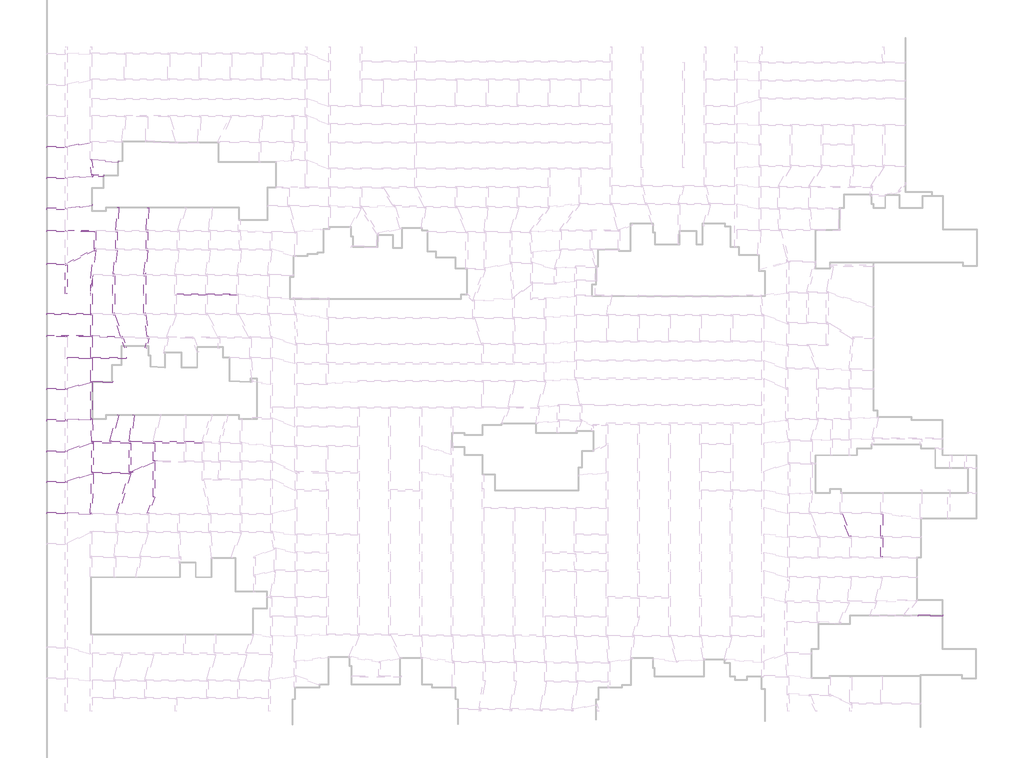
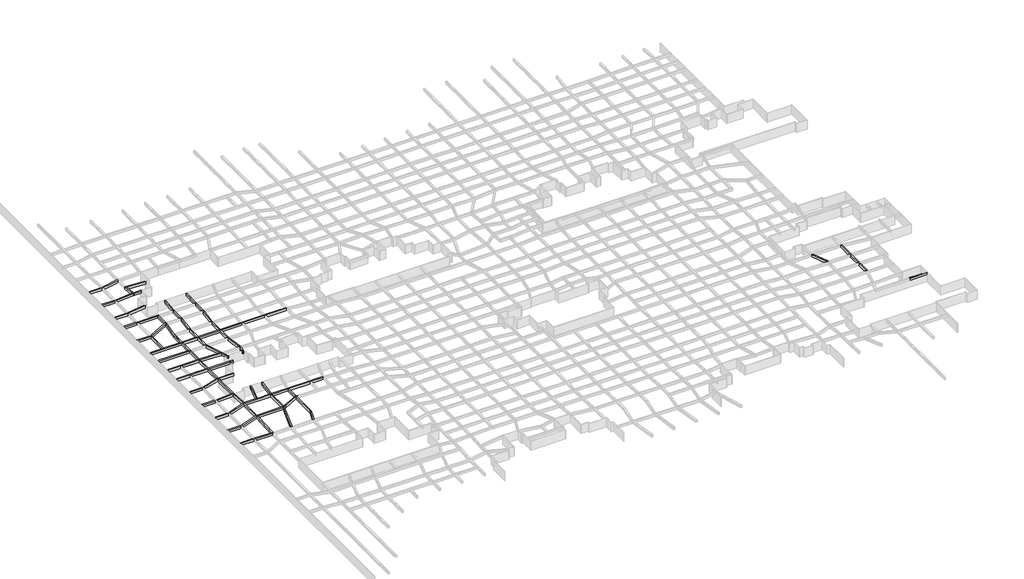
# One storey, part 25 of 45: 64 beams.
"""IFC4 building model written with IfcOpenShell, lengths in millimetres."""

from ifc_helpers import new_model, si_unit, frame, origin, place, context, project, spatial, polyline, outline, extrude, faceted_brep, element, save

model = new_model("IFC4")

# Units and contexts
model_context = context("Model", 3, world=origin())
ifc_project = project(units=[si_unit("LENGTHUNIT", "METRE", prefix="MILLI")], contexts=[model_context])

# Site, building, storey
site = spatial("IfcSite", under=ifc_project)
building = spatial("IfcBuilding", under=site)
storey = spatial("IfcBuildingStorey", under=building, Name="户型图", Elevation=0.0)

# Beams
placement = place(None, origin())
element("IfcBeam", 1, ObjectType="混凝土 - 矩形梁 : KL_beam", at=placement, inside=storey, context=model_context, shape_type="SweptSolid", body=[
    extrude(outline(polyline([(-155040.1872489, 93329.932653), (-155040.1872489, 93729.932653), (-150359.8528414, 93729.932653), (-150359.8528414, 93329.932653), (-155040.1872489, 93329.932653)])), frame((0.0, 0.0, 2500.0), z_axis=(0.0, 0.0, 1.0), x_axis=(1.0, 0.0, 0.0)), (0.0, 0.0, 1.0), 800.0),
])
element("IfcBeam", 2, ObjectType="混凝土 - 矩形梁 : KL_beam", at=placement, inside=storey, context=model_context, shape_type="SweptSolid", body=[
    extrude(outline(polyline([(-155040.1872489, 85529.932653), (-155040.1872489, 85929.932653), (-150359.8528414, 85929.932653), (-150359.8528414, 85529.932653), (-155040.1872489, 85529.932653)])), frame((0.0, 0.0, 2500.0), z_axis=(0.0, 0.0, 1.0), x_axis=(1.0, 0.0, 0.0)), (0.0, 0.0, 1.0), 800.0),
])
element("IfcBeam", 3, ObjectType="混凝土 - 矩形梁 : KL_beam", at=placement, inside=storey, context=model_context, shape_type="SweptSolid", body=[
    extrude(outline(polyline([(-155040.1872489, 77829.932653), (-155040.1872489, 78229.932653), (-150359.8528414, 78229.932653), (-150359.8528414, 77829.932653), (-155040.1872489, 77829.932653)])), frame((0.0, 0.0, 2500.0), z_axis=(0.0, 0.0, 1.0), x_axis=(1.0, 0.0, 0.0)), (0.0, 0.0, 1.0), 800.0),
])
element("IfcBeam", 4, ObjectType="混凝土 - 矩形梁 : KL_beam", at=placement, inside=storey, context=model_context, shape_type="SweptSolid", body=[
    extrude(outline(polyline([(-155040.1872489, 72229.932653), (-155040.1872489, 72629.932653), (-150359.8528414, 72629.932653), (-150359.8528414, 72229.932653), (-155040.1872489, 72229.932653)])), frame((0.0, 0.0, 2500.0), z_axis=(0.0, 0.0, 1.0), x_axis=(1.0, 0.0, 0.0)), (0.0, 0.0, 1.0), 800.0),
])
element("IfcBeam", 5, ObjectType="混凝土 - 矩形梁 : KL_beam", at=placement, inside=storey, context=model_context, shape_type="SweptSolid", body=[
    extrude(outline(polyline([(-155040.1872489, 63929.9626201), (-155040.1872489, 64329.9626201), (-150359.8528414, 64329.9626201), (-150359.8528414, 63929.9626201), (-155040.1872489, 63929.9626201)])), frame((0.0, 0.0, 2500.0), z_axis=(0.0, 0.0, 1.0), x_axis=(1.0, 0.0, 0.0)), (0.0, 0.0, 1.0), 800.0),
])
element("IfcBeam", 6, ObjectType="混凝土 - 矩形梁 : KL_beam", at=placement, inside=storey, context=model_context, shape_type="Brep", body=[
    faceted_brep([(-149959.8528414, 64456.5033467, 3300.0), (-149959.8528414, 64007.5728516, 3300.0), (-143187.4265839, 67458.2963847, 3300.0), (-142895.0186512, 67607.285668, 3300.0), (-142743.034403, 67684.7255104, 3300.0), (-142743.034403, 68007.285668, 3300.0), (-142743.034403, 68133.6560054, 3300.0), (-143143.034403, 67929.8458256, 3300.0), (-149959.8528414, 64007.5728516, 2500.0), (-143187.4265839, 67458.2963847, 2500.0), (-142895.0186512, 67607.285668, 2500.0), (-142743.034403, 67684.7255104, 2500.0), (-149959.8528414, 64456.5033467, 2500.0), (-143143.034403, 67929.8458256, 2500.0), (-142743.034403, 68133.6560054, 2500.0), (-142743.034403, 68007.285668, 2500.0)], [[[0, 1, 2, 3, 4, 5, 6, 7]], [[1, 8, 9, 10, 11, 4, 3, 2]], [[8, 12, 13, 14, 15, 11, 10, 9]], [[6, 14, 13, 12, 0, 7]], [[0, 12, 8, 1]], [[6, 5, 4, 11, 15, 14]]]),
    faceted_brep([(-150359.8528414, 63929.9626201, 3300.0), (-150112.1714971, 63929.9626201, 3300.0), (-150112.1714971, 63929.9626201, 2500.0), (-150359.8528414, 63929.9626201, 2500.0), (-150359.8528414, 63803.7626718, 2500.0), (-150359.8528414, 63803.7626718, 3300.0)], [[[0, 1, 2, 3]], [[4, 5, 0, 3]], [[1, 0, 5]], [[2, 1, 5, 4]], [[3, 2, 4]]]),
])
element("IfcBeam", 7, ObjectType="混凝土 - 矩形梁 : KL_beam", at=placement, inside=storey, context=model_context, shape_type="Brep", body=[
    faceted_brep([(-142743.034403, 72229.932653, 3300.0), (-142743.034403, 72629.6091605, 3300.0), (-142743.034403, 72629.932653, 3300.0), (-149959.8528414, 72629.932653, 3300.0), (-149959.8528414, 72229.932653, 3300.0), (-143143.034403, 72229.932653, 3300.0), (-142743.034403, 72229.932653, 2500.0), (-149959.8528414, 72229.932653, 2500.0), (-143143.034403, 72229.932653, 2500.0), (-142743.034403, 72629.932653, 2500.0), (-142743.034403, 72629.6091605, 2500.0), (-149959.8528414, 72629.932653, 2500.0)], [[[0, 1, 2, 3, 4, 5]], [[6, 0, 5, 4, 7, 8]], [[9, 10, 6, 8, 7, 11]], [[2, 9, 11, 3]], [[4, 3, 11, 7]], [[2, 1, 0, 6, 10, 9]]]),
])
element("IfcBeam", 8, ObjectType="混凝土 - 矩形梁 : KL_beam", at=placement, inside=storey, context=model_context, shape_type="Brep", body=[
    faceted_brep([(-143143.034403, 67929.8458256, 3300.0), (-142743.034403, 68133.6560054, 3300.0), (-142743.034403, 72229.6091605, 3300.0), (-142743.034403, 72229.932653, 3300.0), (-143143.034403, 72229.932653, 3300.0), (-142743.034403, 68133.6560054, 2500.0), (-142743.034403, 72229.6091605, 2500.0), (-142743.034403, 72229.932653, 2500.0), (-143143.034403, 67929.8458256, 2500.0), (-143143.034403, 72229.932653, 2500.0)], [[[0, 1, 2, 3, 4]], [[1, 5, 6, 7, 3, 2]], [[5, 8, 9, 7, 6]], [[8, 0, 4, 9]], [[1, 0, 8, 5]], [[4, 3, 7, 9]]]),
])
element("IfcBeam", 9, ObjectType="混凝土 - 矩形梁 : KL_beam", at=placement, inside=storey, context=model_context, shape_type="SweptSolid", body=[
    extrude(outline(polyline([(-137343.034403, 68007.285668), (-137743.034403, 68007.285668), (-137743.034403, 72229.6091605), (-137343.034403, 72229.6091605), (-137343.034403, 68007.285668)])), frame((0.0, 0.0, 2500.0), z_axis=(0.0, 0.0, 1.0), x_axis=(1.0, 0.0, 0.0)), (0.0, 0.0, 1.0), 800.0),
])
element("IfcBeam", 10, ObjectType="混凝土 - 矩形梁 : KL_beam", at=placement, inside=storey, context=model_context, shape_type="SweptSolid", body=[
    extrude(outline(polyline([(-129643.034403, 68007.285668), (-130043.034403, 68007.285668), (-130043.034403, 72229.6091605), (-129643.034403, 72229.6091605), (-129643.034403, 68007.285668)])), frame((0.0, 0.0, 2500.0), z_axis=(0.0, 0.0, 1.0), x_axis=(1.0, 0.0, 0.0)), (0.0, 0.0, 1.0), 800.0),
])
element("IfcBeam", 11, ObjectType="混凝土 - 矩形梁 : KL_beam", at=placement, inside=storey, context=model_context, shape_type="SweptSolid", body=[
    extrude(outline(polyline([(-129837.0055379, 78332.9949392), (-129437.249207, 78319.0351406), (-129635.9283402, 72629.6091605), (-130036.172158, 72629.6091605), (-129837.0055379, 78332.9949392)])), frame((0.0, 0.0, 2500.0), z_axis=(0.0, 0.0, 1.0), x_axis=(1.0, 0.0, 0.0)), (0.0, 0.0, 1.0), 800.0),
])
element("IfcBeam", 12, ObjectType="混凝土 - 矩形梁 : KL_beam", at=placement, inside=storey, context=model_context, shape_type="SweptSolid", body=[
    extrude(outline(polyline([(-137324.0083706, 78428.9447568), (-136924.9827505, 78401.0421673), (-137328.560661, 72629.6091605), (-137729.5374202, 72629.6091605), (-137324.0083706, 78428.9447568)])), frame((0.0, 0.0, 2500.0), z_axis=(0.0, 0.0, 1.0), x_axis=(1.0, 0.0, 0.0)), (0.0, 0.0, 1.0), 800.0),
])
element("IfcBeam", 13, ObjectType="混凝土 - 矩形梁 : KL_beam", at=placement, inside=storey, context=model_context, shape_type="SweptSolid", body=[
    extrude(outline(polyline([(-143652.5805457, 79146.4826455), (-143596.9113053, 78750.375418), (-149959.8528414, 77856.1223033), (-149959.8528414, 78260.0533323), (-143652.5805457, 79146.4826455)])), frame((0.0, 0.0, 2500.0), z_axis=(0.0, 0.0, 1.0), x_axis=(1.0, 0.0, 0.0)), (0.0, 0.0, 1.0), 800.0),
])
element("IfcBeam", 14, ObjectType="混凝土 - 矩形梁 : KL_beam", at=placement, inside=storey, context=model_context, shape_type="Brep", body=[
    faceted_brep([(-143368.2977458, 86123.352764, 3300.0), (-143401.7015992, 86505.1605551, 3300.0), (-143403.1600429, 86521.8306433, 3300.0), (-143801.6379222, 86486.9683462, 3300.0), (-149959.8528414, 85948.1943532, 3300.0), (-149959.8528414, 85546.6664182, 3300.0), (-143576.2356454, 86105.1605551, 3300.0), (-143368.2977458, 86123.352764, 2500.0), (-149959.8528414, 85546.6664182, 2500.0), (-143576.2356454, 86105.1605551, 2500.0), (-143403.1600429, 86521.8306433, 2500.0), (-143401.7015992, 86505.1605551, 2500.0), (-149959.8528414, 85948.1943532, 2500.0), (-143801.6379222, 86486.9683462, 2500.0)], [[[0, 1, 2, 3, 4, 5, 6]], [[7, 0, 6, 5, 8, 9]], [[10, 11, 7, 9, 8, 12, 13]], [[2, 10, 13, 12, 4, 3]], [[5, 4, 12, 8]], [[2, 1, 0, 7, 11, 10]]]),
])
element("IfcBeam", 15, ObjectType="混凝土 - 矩形梁 : KL_beam", at=placement, inside=storey, context=model_context, shape_type="Brep", body=[
    faceted_brep([(-143749.2394727, 90477.5366261, 3300.0), (-144133.590805, 90443.9102418, 3300.0), (-144147.7173519, 90442.674329, 3300.0), (-143801.6379222, 86486.9683462, 3300.0), (-143403.1600429, 86521.8306433, 3300.0), (-143713.9426126, 90074.09167, 3300.0), (-143749.2394727, 90477.5366261, 2500.0), (-143403.1600429, 86521.8306433, 2500.0), (-143713.9426126, 90074.09167, 2500.0), (-144147.7173519, 90442.674329, 2500.0), (-144133.590805, 90443.9102418, 2500.0), (-143801.6379222, 86486.9683462, 2500.0)], [[[0, 1, 2, 3, 4, 5]], [[6, 0, 5, 4, 7, 8]], [[9, 10, 6, 8, 7, 11]], [[2, 9, 11, 3]], [[4, 3, 11, 7]], [[2, 1, 0, 6, 10, 9]]]),
])
element("IfcBeam", 16, ObjectType="混凝土 - 矩形梁 : KL_beam", at=placement, inside=storey, context=model_context, shape_type="Brep", body=[
    faceted_brep([(-137036.4475634, 90008.1324887, 3300.0), (-137064.3501529, 89609.1068686, 3300.0), (-137064.3501529, 89609.1068686, 2500.0), (-137036.4475634, 90008.1324887, 2500.0), (-143733.590805, 90476.4423647, 3300.0), (-143749.2394727, 90477.5366261, 3300.0), (-143713.9426126, 90074.09167, 3300.0), (-143713.9426126, 90074.09167, 2500.0), (-143749.2394727, 90477.5366261, 2500.0), (-143733.590805, 90476.4423647, 2500.0)], [[[0, 1, 2, 3]], [[1, 0, 4, 5, 6]], [[2, 1, 6, 7]], [[3, 2, 7, 8, 9]], [[0, 3, 9, 8, 5, 4]], [[6, 5, 8, 7]]]),
])
element("IfcBeam", 17, ObjectType="混凝土 - 矩形梁 : KL_beam", at=placement, inside=storey, context=model_context, shape_type="SweptSolid", body=[
    extrude(outline(polyline([(-149959.8528414, 93365.130378), (-149959.8528414, 93772.617056), (-144133.590805, 94905.1276718), (-144133.590805, 94497.6409938), (-149959.8528414, 93365.130378)])), frame((0.0, 0.0, 2500.0), z_axis=(0.0, 0.0, 1.0), x_axis=(1.0, 0.0, 0.0)), (0.0, 0.0, 1.0), 800.0),
])
element("IfcBeam", 18, ObjectType="混凝土 - 矩形梁 : KL_beam", at=placement, inside=storey, context=model_context, shape_type="SweptSolid", body=[
    extrude(outline(polyline([(-140684.967834, 86505.1605551), (-140684.967834, 86105.1605551), (-143576.2356454, 86105.1605551), (-143368.2977458, 86123.352764), (-143401.7015992, 86505.1605551), (-140684.967834, 86505.1605551)])), frame((0.0, 0.0, 2500.0), z_axis=(0.0, 0.0, 1.0), x_axis=(1.0, 0.0, 0.0)), (0.0, 0.0, 1.0), 800.0),
])
element("IfcBeam", 19, ObjectType="混凝土 - 矩形梁 : KL_beam", at=placement, inside=storey, context=model_context, shape_type="SweptSolid", body=[
    extrude(outline(polyline([(-137765.00064, 67607.285668), (-137362.8299892, 67607.285668), (-137992.6084803, 61570.3096597), (-138394.779131, 61570.3096597), (-137765.00064, 67607.285668)])), frame((0.0, 0.0, 2500.0), z_axis=(0.0, 0.0, 1.0), x_axis=(1.0, 0.0, 0.0)), (0.0, 0.0, 1.0), 800.0),
])
element("IfcBeam", 20, ObjectType="混凝土 - 矩形梁 : KL_beam", at=placement, inside=storey, context=model_context, shape_type="Brep", body=[
    faceted_brep([(-129662.8131158, 67607.285668, 3300.0), (-130064.9837666, 67607.285668, 3300.0), (-130694.7622577, 61570.3096597, 3300.0), (-130292.5916069, 61570.3096597, 3300.0), (-130266.1701137, 61823.5827117, 3300.0), (-130064.9837666, 67607.285668, 2500.0), (-130694.7622577, 61570.3096597, 2500.0), (-129662.8131158, 67607.285668, 2500.0), (-130266.1701137, 61823.5827117, 2500.0), (-130292.5916069, 61570.3096597, 2500.0)], [[[0, 1, 2, 3, 4]], [[1, 5, 6, 2]], [[5, 7, 8, 9, 6]], [[7, 0, 4, 3, 9, 8]], [[1, 0, 7, 5]], [[3, 2, 6, 9]]]),
])
element("IfcBeam", 21, ObjectType="混凝土 - 矩形梁 : KL_beam", at=placement, inside=storey, context=model_context, shape_type="Brep", body=[
    faceted_brep([(-130292.5916069, 61570.3096597, 3300.0), (-130266.1701137, 61570.3096597, 3300.0), (-130266.1701137, 61823.5827117, 3300.0), (-130266.1701137, 61570.3096597, 2500.0), (-130266.1701137, 61823.5827117, 2500.0), (-130292.5916069, 61570.3096597, 2500.0)], [[[0, 1, 2]], [[1, 3, 4, 2]], [[3, 5, 4]], [[3, 1, 0, 5]], [[0, 2, 4, 5]]]),
    faceted_brep([(-130266.1701137, 61170.3096597, 3300.0), (-130266.1701137, 61170.3096597, 2500.0), (-130334.3196833, 61170.3096597, 2500.0), (-130666.1701137, 61170.3096597, 2500.0), (-130666.1701137, 61170.3096597, 3300.0), (-130334.3196833, 61170.3096597, 3300.0), (-130666.1701137, 56692.8612022, 3300.0), (-130666.1701137, 56292.8612022, 3300.0), (-130666.1701137, 51854.9299556, 3300.0), (-130266.1701137, 51854.9299556, 3300.0), (-130266.1701137, 56292.8612022, 3300.0), (-130266.1701137, 56692.8612022, 3300.0), (-130266.1701137, 51854.9299556, 2500.0), (-130266.1701137, 56292.8612022, 2500.0), (-130266.1701137, 56692.8612022, 2500.0), (-130666.1701137, 51854.9299556, 2500.0), (-130666.1701137, 56292.8612022, 2500.0), (-130666.1701137, 56692.8612022, 2500.0)], [[[0, 1, 2, 3, 4, 5]], [[5, 4, 6, 7, 8, 9, 10, 11, 0]], [[1, 0, 11, 10, 9, 12, 13, 14]], [[2, 1, 14, 13, 12, 15, 16, 17, 3]], [[4, 3, 17, 16, 15, 8, 7, 6]], [[9, 8, 15, 12]]]),
])
element("IfcBeam", 22, ObjectType="混凝土 - 矩形梁 : KL_beam", at=placement, inside=storey, context=model_context, shape_type="Brep", body=[
    faceted_brep([(-138030.1531976, 61170.3096597, 3300.0), (-138430.1531976, 61170.3096597, 3300.0), (-138430.1531976, 56692.8612022, 3300.0), (-138430.1531976, 56292.8612022, 3300.0), (-138430.1531976, 51854.9299556, 3300.0), (-138030.1531976, 51854.9299556, 3300.0), (-138030.1531976, 56292.8612022, 3300.0), (-138030.1531976, 56692.8612022, 3300.0), (-138030.1531976, 61170.3096597, 2500.0), (-138030.1531976, 51854.9299556, 2500.0), (-138030.1531976, 56292.8612022, 2500.0), (-138030.1531976, 56692.8612022, 2500.0), (-138430.1531976, 61170.3096597, 2500.0), (-138430.1531976, 51854.9299556, 2500.0), (-138430.1531976, 56292.8612022, 2500.0), (-138430.1531976, 56692.8612022, 2500.0)], [[[0, 1, 2, 3, 4, 5, 6, 7]], [[8, 0, 7, 6, 5, 9, 10, 11]], [[12, 8, 11, 10, 9, 13, 14, 15]], [[1, 12, 15, 14, 13, 4, 3, 2]], [[1, 0, 8, 12]], [[5, 4, 13, 9]]]),
])
element("IfcBeam", 23, ObjectType="混凝土 - 矩形梁 : KL_beam", at=placement, inside=storey, context=model_context, shape_type="Brep", body=[
    faceted_brep([(-144029.1794601, 51454.5502515, 2500.0), (-144029.1794601, 51454.5502515, 3300.0), (-144029.1794601, 51854.5502515, 3300.0), (-144029.1794601, 56292.8612022, 3300.0), (-144029.1794601, 56692.8612022, 3300.0), (-144029.1794601, 57320.5657345, 3300.0), (-144029.1794601, 57320.5657345, 2500.0), (-144029.1794601, 56692.8612022, 2500.0), (-144029.1794601, 56292.8612022, 2500.0), (-144029.1794601, 51854.5502515, 2500.0), (-143629.1794601, 51454.5502515, 3300.0), (-143629.1794601, 51454.5502515, 2500.0), (-143629.1794601, 51454.9299556, 3300.0), (-143629.1794601, 51854.9299556, 3300.0), (-143629.1794601, 56292.8612022, 3300.0), (-143629.1794601, 56692.8612022, 3300.0), (-143629.1794601, 60578.3043057, 3300.0), (-143629.1794601, 51454.9299556, 2500.0), (-143629.1794601, 51854.9299556, 2500.0), (-143629.1794601, 56292.8612022, 2500.0), (-143629.1794601, 56692.8612022, 2500.0), (-143629.1794601, 60578.3043057, 2500.0)], [[[0, 1, 2, 3, 4, 5, 6, 7, 8, 9]], [[10, 1, 0, 11]], [[1, 10, 12, 13, 14, 15, 16, 5, 4, 3, 2]], [[10, 11, 17, 18, 19, 20, 21, 16, 15, 14, 13, 12]], [[11, 0, 9, 8, 7, 6, 21, 20, 19, 18, 17]], [[6, 5, 16, 21]]]),
])
element("IfcBeam", 24, ObjectType="混凝土 - 矩形梁 : KL_beam", at=placement, inside=storey, context=model_context, shape_type="Brep", body=[
    faceted_brep([(-155040.3480617, 56292.8612022, 3300.0), (-155040.3480617, 56692.8612022, 3300.0), (-155040.3480617, 56692.8612022, 2500.0), (-155040.3480617, 56292.8612022, 2500.0), (-144029.1794601, 56292.8612022, 3300.0), (-144029.1794601, 56692.8612022, 3300.0), (-149959.8528414, 56692.8612022, 3300.0), (-150359.8528414, 56692.8612022, 3300.0), (-144029.1794601, 56692.8612022, 2500.0), (-149959.8528414, 56692.8612022, 2500.0), (-150359.8528414, 56692.8612022, 2500.0), (-144029.1794601, 56292.8612022, 2500.0)], [[[0, 1, 2, 3]], [[1, 0, 4, 5, 6, 7]], [[2, 1, 7, 6, 5, 8, 9, 10]], [[3, 2, 10, 9, 8, 11]], [[0, 3, 11, 4]], [[5, 4, 11, 8]]]),
    faceted_brep([(-107154.3480617, 56292.8612022, 3300.0), (-107154.3480617, 56292.8612022, 2500.0), (-107154.3480617, 56670.8773262, 2500.0), (-107154.3480617, 56692.8612022, 2500.0), (-107154.3480617, 56692.8612022, 3300.0), (-107154.3480617, 56670.8773262, 3300.0), (-122502.1870297, 56292.8612022, 3300.0), (-122502.1870297, 56692.8612022, 3300.0), (-122502.1870297, 56692.8612022, 2500.0), (-122502.1870297, 56292.8612022, 2500.0), (-114728.2029549, 56692.8612022, 3300.0), (-115128.2029549, 56692.8612022, 3300.0), (-115128.2029549, 56292.8612022, 3300.0), (-114728.2029549, 56292.8612022, 3300.0), (-107385.8902631, 56292.8612022, 3300.0), (-114728.2029549, 56692.8612022, 2500.0), (-115128.2029549, 56692.8612022, 2500.0), (-107385.8902631, 56292.8612022, 2500.0), (-114728.2029549, 56292.8612022, 2500.0), (-115128.2029549, 56292.8612022, 2500.0)], [[[0, 1, 2, 3, 4, 5]], [[6, 7, 8, 9]], [[0, 5, 4, 10, 11, 7, 6, 12, 13, 14]], [[4, 3, 15, 16, 8, 7, 11, 10]], [[3, 2, 1, 17, 18, 19, 9, 8, 16, 15]], [[1, 0, 14, 13, 12, 6, 9, 19, 18, 17]]]),
    faceted_brep([(-122902.1870297, 56692.8612022, 3300.0), (-122902.1870297, 56292.8612022, 3300.0), (-122902.1870297, 56292.8612022, 2500.0), (-122902.1870297, 56692.8612022, 2500.0), (-130266.1701137, 56292.8612022, 3300.0), (-130266.1701137, 56692.8612022, 3300.0), (-130266.1701137, 56692.8612022, 2500.0), (-130266.1701137, 56292.8612022, 2500.0)], [[[0, 1, 2, 3]], [[4, 5, 6, 7]], [[1, 0, 5, 4]], [[0, 3, 6, 5]], [[3, 2, 7, 6]], [[2, 1, 4, 7]]]),
    faceted_brep([(-130666.1701137, 56692.8612022, 3300.0), (-130666.1701137, 56292.8612022, 3300.0), (-130666.1701137, 56292.8612022, 2500.0), (-130666.1701137, 56692.8612022, 2500.0), (-138030.1531976, 56292.8612022, 3300.0), (-138030.1531976, 56692.8612022, 3300.0), (-138030.1531976, 56692.8612022, 2500.0), (-138030.1531976, 56292.8612022, 2500.0)], [[[0, 1, 2, 3]], [[4, 5, 6, 7]], [[1, 0, 5, 4]], [[0, 3, 6, 5]], [[3, 2, 7, 6]], [[2, 1, 4, 7]]]),
    faceted_brep([(-138430.1531976, 56692.8612022, 3300.0), (-138430.1531976, 56292.8612022, 3300.0), (-138430.1531976, 56292.8612022, 2500.0), (-138430.1531976, 56692.8612022, 2500.0), (-143629.1794601, 56292.8612022, 3300.0), (-143629.1794601, 56692.8612022, 3300.0), (-143629.1794601, 56692.8612022, 2500.0), (-143629.1794601, 56292.8612022, 2500.0)], [[[0, 1, 2, 3]], [[4, 5, 6, 7]], [[1, 0, 5, 4]], [[0, 3, 6, 5]], [[3, 2, 7, 6]], [[2, 1, 4, 7]]]),
])
element("IfcBeam", 25, ObjectType="混凝土 - 矩形梁 : KL_beam", at=placement, inside=storey, context=model_context, shape_type="SweptSolid", body=[
    extrude(outline(polyline([(-149959.8528414, 63929.9626201), (-149959.8528414, 56692.8612022), (-150359.8528414, 56692.8612022), (-150359.8528414, 63803.7626718), (-150112.1714971, 63929.9626201), (-149959.8528414, 63929.9626201)])), frame((0.0, 0.0, 2500.0), z_axis=(0.0, 0.0, 1.0), x_axis=(1.0, 0.0, 0.0)), (0.0, 0.0, 1.0), 800.0),
])
element("IfcBeam", 26, ObjectType="混凝土 - 矩形梁 : KL_beam", at=placement, inside=storey, context=model_context, shape_type="SweptSolid", body=[
    extrude(outline(polyline([(-155040.3505583, 51454.5502515), (-155040.3505583, 51854.5502515), (-144029.1794601, 51854.5502515), (-144029.1794601, 51454.5502515), (-155040.3505583, 51454.5502515)])), frame((0.0, 0.0, 2500.0), z_axis=(0.0, 0.0, 1.0), x_axis=(1.0, 0.0, 0.0)), (0.0, 0.0, 1.0), 800.0),
])
element("IfcBeam", 27, ObjectType="混凝土 - 矩形梁 : KL_beam", at=placement, inside=storey, context=model_context, shape_type="SweptSolid", body=[
    extrude(outline(polyline([(-130640.0234877, 51454.9299556), (-130236.0924587, 51454.9299556), (-129458.8661012, 45924.6770642), (-129862.7971302, 45924.6770642), (-130640.0234877, 51454.9299556)])), frame((0.0, 0.0, 2500.0), z_axis=(0.0, 0.0, 1.0), x_axis=(1.0, 0.0, 0.0)), (0.0, 0.0, 1.0), 800.0),
])
element("IfcBeam", 28, ObjectType="混凝土 - 矩形梁 : KL_beam", at=placement, inside=storey, context=model_context, shape_type="SweptSolid", body=[
    extrude(outline(polyline([(-135993.089329, 45924.6770642), (-136417.3284341, 45924.6770642), (-138371.532439, 51454.9299556), (-137947.2933339, 51454.9299556), (-135993.089329, 45924.6770642)])), frame((0.0, 0.0, 2500.0), z_axis=(0.0, 0.0, 1.0), x_axis=(1.0, 0.0, 0.0)), (0.0, 0.0, 1.0), 800.0),
])
element("IfcBeam", 29, ObjectType="混凝土 - 矩形梁 : KL_beam", at=placement, inside=storey, context=model_context, shape_type="Brep", body=[
    faceted_brep([(-144029.1794601, 25141.8814872, 3300.0), (-144018.8658517, 25142.5337653, 3300.0), (-143629.1794601, 25167.1792512, 3300.0), (-143629.1794601, 25366.7986539, 3300.0), (-143629.1794601, 34369.9375221, 3300.0), (-143629.1794601, 34769.9375221, 3300.0), (-143629.1794601, 40354.5502515, 3300.0), (-143629.1794601, 40754.5502515, 3300.0), (-143629.1794601, 45845.780438, 3300.0), (-143629.1794601, 46246.148229, 3300.0), (-143629.1794601, 51454.5502515, 3300.0), (-144029.1794601, 51454.5502515, 3300.0), (-144029.1794601, 46254.5502515, 3300.0), (-144029.1794601, 45854.5502515, 3300.0), (-144029.1794601, 40754.5502515, 3300.0), (-144029.1794601, 40354.5502515, 3300.0), (-144029.1794601, 34720.6483321, 3300.0), (-144029.1794601, 34304.5285578, 3300.0), (-144029.1794601, 25542.6806599, 3300.0), (-144029.1794601, 25141.8814872, 2500.0), (-144029.1794601, 51454.5502515, 2500.0), (-144029.1794601, 46254.5502515, 2500.0), (-144029.1794601, 45854.5502515, 2500.0), (-144029.1794601, 40754.5502515, 2500.0), (-144029.1794601, 40354.5502515, 2500.0), (-144029.1794601, 34720.6483321, 2500.0), (-144029.1794601, 34304.5285578, 2500.0), (-144029.1794601, 25542.6806599, 2500.0), (-143629.1794601, 25167.1792512, 2500.0), (-144018.8658517, 25142.5337653, 2500.0), (-143629.1794601, 51454.5502515, 2500.0), (-143629.1794601, 46246.148229, 2500.0), (-143629.1794601, 45845.780438, 2500.0), (-143629.1794601, 40754.5502515, 2500.0), (-143629.1794601, 40354.5502515, 2500.0), (-143629.1794601, 34769.9375221, 2500.0), (-143629.1794601, 34369.9375221, 2500.0), (-143629.1794601, 25366.7986539, 2500.0)], [[[0, 1, 2, 3, 4, 5, 6, 7, 8, 9, 10, 11, 12, 13, 14, 15, 16, 17, 18]], [[19, 0, 18, 17, 16, 15, 14, 13, 12, 11, 20, 21, 22, 23, 24, 25, 26, 27]], [[28, 29, 19, 27, 26, 25, 24, 23, 22, 21, 20, 30, 31, 32, 33, 34, 35, 36, 37]], [[2, 28, 37, 36, 35, 34, 33, 32, 31, 30, 10, 9, 8, 7, 6, 5, 4, 3]], [[11, 10, 30, 20]], [[2, 1, 0, 19, 29, 28]]]),
])
element("IfcBeam", 30, ObjectType="混凝土 - 矩形梁 : KL_beam", at=placement, inside=storey, context=model_context, shape_type="Brep", body=[
    faceted_brep([(-155040.3505583, 46254.5502515, 3300.0), (-155040.3505583, 46254.5502515, 2500.0), (-155040.3505583, 45854.5502515, 2500.0), (-155040.3505583, 45854.5502515, 3300.0), (-150359.8528414, 45854.5502515, 3300.0), (-149959.8528414, 45854.5502515, 3300.0), (-144029.1794601, 45854.5502515, 3300.0), (-144029.1794601, 46254.5502515, 3300.0), (-150359.8528414, 45854.5502515, 2500.0), (-149959.8528414, 45854.5502515, 2500.0), (-144029.1794601, 45854.5502515, 2500.0), (-144029.1794601, 46254.5502515, 2500.0)], [[[0, 1, 2, 3]], [[0, 3, 4, 5, 6, 7]], [[3, 2, 8, 9, 10, 6, 5, 4]], [[2, 1, 11, 10, 9, 8]], [[1, 0, 7, 11]], [[7, 6, 10, 11]]]),
])
element("IfcBeam", 31, ObjectType="混凝土 - 矩形梁 : KL_beam", at=placement, inside=storey, context=model_context, shape_type="SweptSolid", body=[
    extrude(outline(polyline([(-136126.2918172, 45924.3276551), (-136143.4332141, 45524.6951082), (-143629.1794601, 45845.780438), (-143629.1794601, 46246.148229), (-136126.2918172, 45924.3276551)])), frame((0.0, 0.0, 2500.0), z_axis=(0.0, 0.0, 1.0), x_axis=(1.0, 0.0, 0.0)), (0.0, 0.0, 1.0), 800.0),
])
element("IfcBeam", 32, ObjectType="混凝土 - 矩形梁 : KL_beam", at=placement, inside=storey, context=model_context, shape_type="SweptSolid", body=[
    extrude(outline(polyline([(-155040.3505583, 40354.5502515), (-155040.3505583, 40754.5502515), (-150359.8528414, 40754.5502515), (-150359.8528414, 40354.5502515), (-155040.3505583, 40354.5502515)])), frame((0.0, 0.0, 2500.0), z_axis=(0.0, 0.0, 1.0), x_axis=(1.0, 0.0, 0.0)), (0.0, 0.0, 1.0), 800.0),
    extrude(outline(polyline([(-144029.1794601, 40754.5502515), (-144029.1794601, 40354.5502515), (-149959.8528414, 40354.5502515), (-149959.8528414, 40754.5502515), (-144029.1794601, 40754.5502515)])), frame((0.0, 0.0, 2500.0), z_axis=(0.0, 0.0, 1.0), x_axis=(1.0, 0.0, 0.0)), (0.0, 0.0, 1.0), 800.0),
])
element("IfcBeam", 33, ObjectType="混凝土 - 矩形梁 : KL_beam", at=placement, inside=storey, context=model_context, shape_type="SweptSolid", body=[
    extrude(outline(polyline([(-135130.1663289, 40754.5502515), (-135130.1663289, 40354.5502515), (-143629.1794601, 40354.5502515), (-143629.1794601, 40754.5502515), (-135130.1663289, 40754.5502515)])), frame((0.0, 0.0, 2500.0), z_axis=(0.0, 0.0, 1.0), x_axis=(1.0, 0.0, 0.0)), (0.0, 0.0, 1.0), 800.0),
])
element("IfcBeam", 34, ObjectType="混凝土 - 矩形梁 : KL_beam", at=placement, inside=storey, context=model_context, shape_type="SweptSolid", body=[
    extrude(outline(polyline([(-155040.1872489, 32554.5502515), (-155040.1872489, 32954.5502515), (-150359.8528414, 32954.5502515), (-150359.8528414, 32554.5502515), (-155040.1872489, 32554.5502515)])), frame((0.0, 0.0, 2500.0), z_axis=(0.0, 0.0, 1.0), x_axis=(1.0, 0.0, 0.0)), (0.0, 0.0, 1.0), 800.0),
])
element("IfcBeam", 35, ObjectType="混凝土 - 矩形梁 : KL_beam", at=placement, inside=storey, context=model_context, shape_type="SweptSolid", body=[
    extrude(outline(polyline([(-144029.1794601, 34720.6483321), (-144029.1794601, 34304.5285578), (-149959.8528414, 32603.9353313), (-149959.8528414, 33020.0551056), (-144029.1794601, 34720.6483321)])), frame((0.0, 0.0, 2500.0), z_axis=(0.0, 0.0, 1.0), x_axis=(1.0, 0.0, 0.0)), (0.0, 0.0, 1.0), 800.0),
])
element("IfcBeam", 36, ObjectType="混凝土 - 矩形梁 : KL_beam", at=placement, inside=storey, context=model_context, shape_type="SweptSolid", body=[
    extrude(outline(polyline([(-138429.1794601, 34769.9375221), (-138429.1794601, 34369.9375221), (-143629.1794601, 34369.9375221), (-143629.1794601, 34769.9375221), (-138429.1794601, 34769.9375221)])), frame((0.0, 0.0, 2500.0), z_axis=(0.0, 0.0, 1.0), x_axis=(1.0, 0.0, 0.0)), (0.0, 0.0, 1.0), 800.0),
])
element("IfcBeam", 37, ObjectType="混凝土 - 矩形梁 : KL_beam", at=placement, inside=storey, context=model_context, shape_type="SweptSolid", body=[
    extrude(outline(polyline([(-155040.1872489, 24754.5502515), (-155040.1872489, 25154.5502515), (-150359.8528414, 25154.5502515), (-150359.8528414, 24754.5502515), (-155040.1872489, 24754.5502515)])), frame((0.0, 0.0, 2500.0), z_axis=(0.0, 0.0, 1.0), x_axis=(1.0, 0.0, 0.0)), (0.0, 0.0, 1.0), 800.0),
])
element("IfcBeam", 38, ObjectType="混凝土 - 矩形梁 : KL_beam", at=placement, inside=storey, context=model_context, shape_type="SweptSolid", body=[
    extrude(outline(polyline([(-144029.1794601, 25542.6806599), (-144029.1794601, 25141.8814872), (-149959.8528414, 24766.7995471), (-149959.8528414, 25167.5987199), (-144029.1794601, 25542.6806599)])), frame((0.0, 0.0, 2500.0), z_axis=(0.0, 0.0, 1.0), x_axis=(1.0, 0.0, 0.0)), (0.0, 0.0, 1.0), 800.0),
])
element("IfcBeam", 39, ObjectType="混凝土 - 矩形梁 : KL_beam", at=placement, inside=storey, context=model_context, shape_type="SweptSolid", body=[
    extrude(outline(polyline([(-155040.1872489, 16954.5502515), (-155040.1872489, 17354.5502515), (-150359.8528414, 17354.5502515), (-150359.8528414, 16954.5502515), (-155040.1872489, 16954.5502515)])), frame((0.0, 0.0, 2500.0), z_axis=(0.0, 0.0, 1.0), x_axis=(1.0, 0.0, 0.0)), (0.0, 0.0, 1.0), 800.0),
])
element("IfcBeam", 40, ObjectType="混凝土 - 矩形梁 : KL_beam", at=placement, inside=storey, context=model_context, shape_type="Brep", body=[
    faceted_brep([(-143344.2950634, 19289.9260039, 3300.0), (-143474.5223252, 19668.1334341, 3300.0), (-143751.2646427, 19572.8434125, 3300.0), (-149959.8528414, 17435.0550561, 3300.0), (-149959.8528414, 17012.0067836, 3300.0), (-143744.2950635, 19152.1949586, 3300.0), (-143344.2950634, 19289.9260039, 2500.0), (-149959.8528414, 17012.0067836, 2500.0), (-143744.2950635, 19152.1949586, 2500.0), (-143474.5223252, 19668.1334341, 2500.0), (-149959.8528414, 17435.0550561, 2500.0), (-143751.2646427, 19572.8434125, 2500.0)], [[[0, 1, 2, 3, 4, 5]], [[6, 0, 5, 4, 7, 8]], [[9, 6, 8, 7, 10, 11]], [[1, 9, 11, 10, 3, 2]], [[4, 3, 10, 7]], [[1, 0, 6, 9]]]),
])
element("IfcBeam", 41, ObjectType="混凝土 - 矩形梁 : KL_beam", at=placement, inside=storey, context=model_context, shape_type="SweptSolid", body=[
    extrude(outline(polyline([(-155040.1872489, 9254.5502515), (-155040.1872489, 9654.5502515), (-150359.8528414, 9654.5502515), (-150359.8528414, 9254.5502515), (-155040.1872489, 9254.5502515)])), frame((0.0, 0.0, 2500.0), z_axis=(0.0, 0.0, 1.0), x_axis=(1.0, 0.0, 0.0)), (0.0, 0.0, 1.0), 800.0),
])
element("IfcBeam", 42, ObjectType="混凝土 - 矩形梁 : KL_beam", at=placement, inside=storey, context=model_context, shape_type="Brep", body=[
    faceted_brep([(-143349.4497455, 11588.0359588, 3300.0), (-143479.6770073, 11966.243389, 3300.0), (-143744.2950635, 11875.1280853, 3300.0), (-149959.8528414, 9734.9399104, 3300.0), (-149959.8528414, 9311.8916379, 3300.0), (-143754.5647409, 11448.5436793, 3300.0), (-143349.4497455, 11588.0359588, 2500.0), (-149959.8528414, 9311.8916379, 2500.0), (-143754.5647409, 11448.5436793, 2500.0), (-143479.6770073, 11966.243389, 2500.0), (-149959.8528414, 9734.9399104, 2500.0), (-143744.2950635, 11875.1280853, 2500.0)], [[[0, 1, 2, 3, 4, 5]], [[6, 0, 5, 4, 7, 8]], [[9, 6, 8, 7, 10, 11]], [[1, 9, 11, 10, 3, 2]], [[4, 3, 10, 7]], [[1, 0, 6, 9]]]),
])
element("IfcBeam", 43, ObjectType="混凝土 - 矩形梁 : KL_beam", at=placement, inside=storey, context=model_context, shape_type="SweptSolid", body=[
    extrude(outline(polyline([(-155040.1872489, 1454.5502515), (-155040.1872489, 1854.5502515), (-150359.8528414, 1854.5502515), (-150359.8528414, 1454.5502515), (-155040.1872489, 1454.5502515)])), frame((0.0, 0.0, 2500.0), z_axis=(0.0, 0.0, 1.0), x_axis=(1.0, 0.0, 0.0)), (0.0, 0.0, 1.0), 800.0),
])
element("IfcBeam", 44, ObjectType="混凝土 - 矩形梁 : KL_beam", at=placement, inside=storey, context=model_context, shape_type="Brep", body=[
    faceted_brep([(-143704.0852782, 1228.9879716, 3300.0), (-143704.0852782, 1432.6030214, 3300.0), (-143704.0852782, 1629.2317894, 3300.0), (-144096.9835442, 1642.9520991, 3300.0), (-149959.8528414, 1847.6880064, 3300.0), (-149959.8528414, 1447.4441887, 3300.0), (-144104.0852782, 1242.9562794, 3300.0), (-143704.0852782, 1228.9879716, 2500.0), (-149959.8528414, 1447.4441887, 2500.0), (-144104.0852782, 1242.9562794, 2500.0), (-143704.0852782, 1629.2317894, 2500.0), (-143704.0852782, 1432.6030214, 2500.0), (-149959.8528414, 1847.6880064, 2500.0), (-144096.9835442, 1642.9520991, 2500.0)], [[[0, 1, 2, 3, 4, 5, 6]], [[7, 0, 6, 5, 8, 9]], [[10, 11, 7, 9, 8, 12, 13]], [[2, 10, 13, 12, 4, 3]], [[5, 4, 12, 8]], [[2, 1, 0, 7, 11, 10]]]),
])
element("IfcBeam", 45, ObjectType="混凝土 - 矩形梁 : KL_beam", at=placement, inside=storey, context=model_context, shape_type="Brep", body=[
    faceted_brep([(-143349.4497455, 11588.0359588, 3300.0), (-143754.5647409, 11448.5436793, 3300.0), (-144096.9835442, 1642.9520991, 3300.0), (-143704.0852782, 1629.2317894, 3300.0), (-143704.0852782, 1432.6030214, 3300.0), (-143698.467803, 1593.466462, 3300.0), (-143351.4029561, 11532.1033248, 3300.0), (-143349.4497455, 11588.0359588, 2500.0), (-143704.0852782, 1432.6030214, 2500.0), (-143698.467803, 1593.466462, 2500.0), (-143351.4029561, 11532.1033248, 2500.0), (-143754.5647409, 11448.5436793, 2500.0), (-143704.0852782, 1629.2317894, 2500.0), (-144096.9835442, 1642.9520991, 2500.0)], [[[0, 1, 2, 3, 4, 5, 6]], [[7, 0, 6, 5, 4, 8, 9, 10]], [[11, 7, 10, 9, 8, 12, 13]], [[1, 11, 13, 2]], [[1, 0, 7, 11]], [[12, 3, 2, 13]], [[3, 12, 8, 4]]]),
])
element("IfcBeam", 46, ObjectType="混凝土 - 矩形梁 : KL_beam", at=placement, inside=storey, context=model_context, shape_type="Brep", body=[
    faceted_brep([(-143344.2950634, 19289.9260039, 3300.0), (-143744.2950635, 19152.1949586, 3300.0), (-143744.2950635, 11875.1280853, 3300.0), (-143739.6117725, 11876.7406717, 3300.0), (-143479.6770073, 11966.243389, 3300.0), (-143349.4497455, 11588.0359588, 3300.0), (-143351.4029561, 11532.1033248, 3300.0), (-143344.2950635, 11532.1033248, 3300.0), (-143344.2950635, 11932.1033248, 3300.0), (-143344.2950634, 19232.6251957, 3300.0), (-143344.2950634, 19289.9260039, 2500.0), (-143344.2950635, 11532.1033248, 2500.0), (-143344.2950635, 11932.1033248, 2500.0), (-143344.2950634, 19232.6251957, 2500.0), (-143744.2950635, 19152.1949586, 2500.0), (-143351.4029561, 11532.1033248, 2500.0), (-143349.4497455, 11588.0359588, 2500.0), (-143479.6770073, 11966.243389, 2500.0), (-143739.6117725, 11876.7406717, 2500.0), (-143744.2950635, 11875.1280853, 2500.0)], [[[0, 1, 2, 3, 4, 5, 6, 7, 8, 9]], [[10, 0, 9, 8, 7, 11, 12, 13]], [[14, 10, 13, 12, 11, 15, 16, 17, 18, 19]], [[1, 14, 19, 2]], [[1, 0, 10, 14]], [[17, 4, 3, 2, 19, 18]], [[4, 17, 16, 5]], [[11, 7, 6, 15]], [[6, 5, 16, 15]]]),
])
element("IfcBeam", 47, ObjectType="混凝土 - 矩形梁 : KL_beam", at=placement, inside=storey, context=model_context, shape_type="Brep", body=[
    faceted_brep([(-143344.2950635, 19437.3864455, 3300.0), (-143344.2950635, 19437.3864455, 2500.0), (-143353.6754998, 19632.6251957, 2500.0), (-143629.1794601, 25366.7986539, 2500.0), (-143629.1794601, 25366.7986539, 3300.0), (-143353.6754998, 19632.6251957, 3300.0), (-143344.2950634, 19289.9260039, 3300.0), (-143344.2950634, 19289.9260039, 2500.0), (-143474.5223252, 19668.1334341, 2500.0), (-143474.5223252, 19668.1334341, 3300.0), (-143744.2950635, 19575.2432311, 3300.0), (-143751.2646427, 19572.8434125, 3300.0), (-143751.2646427, 19572.8434125, 2500.0), (-143744.2950635, 19575.2432311, 2500.0), (-143629.1794601, 25167.1792512, 2500.0), (-143629.1794601, 25167.1792512, 3300.0), (-144018.8658517, 25142.5337653, 2500.0), (-144018.8658517, 25142.5337653, 3300.0)], [[[0, 1, 2, 3, 4, 5]], [[0, 6, 7, 1]], [[8, 9, 10, 11, 12, 13]], [[9, 8, 7, 6]], [[14, 15, 4, 3]], [[15, 14, 16, 17]], [[6, 0, 5, 4, 15, 17, 11, 10, 9]], [[1, 7, 8, 13, 12, 16, 14, 3, 2]], [[12, 11, 17, 16]]]),
])
element("IfcBeam", 48, ObjectType="混凝土 - 矩形梁 : KL_beam", at=placement, inside=storey, context=model_context, shape_type="Brep", body=[
    faceted_brep([(-115838.9400314, 19632.6251957, 3300.0), (-115992.1694307, 19632.6251957, 3300.0), (-120144.2950634, 19632.6251957, 3300.0), (-120544.2950634, 19632.6251957, 3300.0), (-127897.3156321, 19632.6251957, 3300.0), (-128306.2518701, 19632.6251957, 3300.0), (-133918.2361862, 19632.6251957, 3300.0), (-134321.2401164, 19632.6251957, 3300.0), (-138783.6499889, 19632.6251957, 3300.0), (-139197.760461, 19632.6251957, 3300.0), (-143353.6754998, 19632.6251957, 3300.0), (-143344.2950634, 19437.3864455, 3300.0), (-143344.2950634, 19289.9260039, 3300.0), (-143344.2950634, 19232.6251957, 3300.0), (-134344.2950634, 19232.6251957, 3300.0), (-133944.2950634, 19232.6251957, 3300.0), (-128344.2950634, 19232.6251957, 3300.0), (-127944.2950634, 19232.6251957, 3300.0), (-120544.2950634, 19232.6251957, 3300.0), (-120144.2950634, 19232.6251957, 3300.0), (-116044.2371144, 19232.6251957, 3300.0), (-115849.4144, 19232.6251957, 3300.0), (-115849.4144, 19232.6251957, 2500.0), (-143344.2950634, 19232.6251957, 2500.0), (-134344.2950634, 19232.6251957, 2500.0), (-133944.2950634, 19232.6251957, 2500.0), (-128344.2950634, 19232.6251957, 2500.0), (-127944.2950634, 19232.6251957, 2500.0), (-120544.2950634, 19232.6251957, 2500.0), (-120144.2950634, 19232.6251957, 2500.0), (-116044.2371144, 19232.6251957, 2500.0), (-143353.6754998, 19632.6251957, 2500.0), (-139197.760461, 19632.6251957, 2500.0), (-138783.6499889, 19632.6251957, 2500.0), (-134321.2401164, 19632.6251957, 2500.0), (-133918.2361862, 19632.6251957, 2500.0), (-128306.2518701, 19632.6251957, 2500.0), (-127897.3156321, 19632.6251957, 2500.0), (-120544.2950634, 19632.6251957, 2500.0), (-120144.2950634, 19632.6251957, 2500.0), (-115992.1694307, 19632.6251957, 2500.0), (-115838.9400314, 19632.6251957, 2500.0), (-143344.2950634, 19289.9260039, 2500.0), (-143344.2950634, 19437.3864455, 2500.0)], [[[0, 1, 2, 3, 4, 5, 6, 7, 8, 9, 10, 11, 12, 13, 14, 15, 16, 17, 18, 19, 20, 21]], [[22, 21, 20, 19, 18, 17, 16, 15, 14, 13, 23, 24, 25, 26, 27, 28, 29, 30]], [[31, 32, 33, 34, 35, 36, 37, 38, 39, 40, 41, 22, 30, 29, 28, 27, 26, 25, 24, 23, 42, 43]], [[10, 9, 8, 7, 6, 5, 4, 3, 2, 1, 0, 41, 40, 39, 38, 37, 36, 35, 34, 33, 32, 31]], [[43, 11, 10, 31]], [[11, 43, 42, 23, 13, 12]], [[0, 21, 22, 41]]]),
])
element("IfcBeam", 49, ObjectType="混凝土 - 矩形梁 : KL_beam", at=placement, inside=storey, context=model_context, shape_type="Brep", body=[
    faceted_brep([(-143344.2950634, 11932.1033248, 3300.0), (-143344.2950635, 11532.1033248, 3300.0), (-134415.3909629, 11532.1033248, 3300.0), (-134098.744249, 11532.1033248, 3300.0), (-133979.3039407, 11590.3582556, 3300.0), (-133278.6227124, 11932.1033248, 3300.0), (-134191.0915255, 11932.1033248, 3300.0), (-134344.2950634, 11932.1033248, 3300.0), (-143344.2950635, 11532.1033248, 2500.0), (-134415.3909629, 11532.1033248, 2500.0), (-134098.744249, 11532.1033248, 2500.0), (-143344.2950634, 11932.1033248, 2500.0), (-134344.2950634, 11932.1033248, 2500.0), (-134191.0915255, 11932.1033248, 2500.0), (-133278.6227124, 11932.1033248, 2500.0), (-133979.3039407, 11590.3582556, 2500.0)], [[[0, 1, 2, 3, 4, 5, 6, 7]], [[1, 8, 9, 10, 3, 2]], [[8, 11, 12, 13, 14, 15, 10, 9]], [[11, 0, 7, 6, 5, 14, 13, 12]], [[1, 0, 11, 8]], [[5, 4, 3, 10, 15, 14]]]),
])
element("IfcBeam", 50, ObjectType="混凝土 - 矩形梁 : KL_beam", at=placement, inside=storey, context=model_context, shape_type="Brep", body=[
    faceted_brep([(-127346.5820068, 14825.3528936, 3300.0), (-127944.2950634, 14825.3528936, 3300.0), (-128259.0508199, 14825.3528936, 3300.0), (-128344.2950634, 14783.776498, 3300.0), (-133944.2950634, 12052.4740021, 3300.0), (-134191.0915255, 11932.1033248, 3300.0), (-133278.6227124, 11932.1033248, 3300.0), (-128344.2950634, 14338.7357219, 3300.0), (-128166.7035435, 14425.3528936, 3300.0), (-127346.5820068, 14825.3528936, 2500.0), (-133278.6227124, 11932.1033248, 2500.0), (-128344.2950634, 14338.7357219, 2500.0), (-128166.7035435, 14425.3528936, 2500.0), (-128259.0508199, 14825.3528936, 2500.0), (-127944.2950634, 14825.3528936, 2500.0), (-134191.0915255, 11932.1033248, 2500.0), (-133944.2950634, 12052.4740021, 2500.0), (-128344.2950634, 14783.776498, 2500.0)], [[[0, 1, 2, 3, 4, 5, 6, 7, 8]], [[9, 0, 8, 7, 6, 10, 11, 12]], [[13, 14, 9, 12, 11, 10, 15, 16, 17]], [[2, 13, 17, 16, 15, 5, 4, 3]], [[6, 5, 15, 10]], [[2, 1, 0, 9, 14, 13]]]),
])
element("IfcBeam", 51, ObjectType="混凝土 - 矩形梁 : KL_beam", at=placement, inside=storey, context=model_context, shape_type="SweptSolid", body=[
    extrude(outline(polyline([(-134344.2950634, 19232.6251957), (-133944.2950634, 19232.6251957), (-133944.2950634, 12052.4740021), (-134191.0915255, 11932.1033248), (-134344.2950634, 11932.1033248), (-134344.2950634, 19232.6251957)])), frame((0.0, 0.0, 2500.0), z_axis=(0.0, 0.0, 1.0), x_axis=(1.0, 0.0, 0.0)), (0.0, 0.0, 1.0), 800.0),
])
element("IfcBeam", 52, ObjectType="混凝土 - 矩形梁 : KL_beam", at=placement, inside=storey, context=model_context, shape_type="SweptSolid", body=[
    extrude(outline(polyline([(-128344.2950634, 19232.6251957), (-127944.2950634, 19232.6251957), (-127944.2950634, 14825.3528936), (-128259.0508199, 14825.3528936), (-128344.2950634, 14783.776498), (-128344.2950634, 19232.6251957)])), frame((0.0, 0.0, 2500.0), z_axis=(0.0, 0.0, 1.0), x_axis=(1.0, 0.0, 0.0)), (0.0, 0.0, 1.0), 800.0),
])
element("IfcBeam", 53, ObjectType="混凝土 - 矩形梁 : KL_beam", at=placement, inside=storey, context=model_context, shape_type="Brep", body=[
    faceted_brep([(-144029.1794601, 60602.7693538, 3300.0), (-144029.1794601, 57320.5657345, 3300.0), (-143629.1794601, 60578.3043057, 3300.0), (-143556.4903427, 61170.3096597, 3300.0), (-143507.3765183, 61570.3096597, 3300.0), (-142766.12907, 67607.285668, 3300.0), (-142895.0186512, 67607.285668, 3300.0), (-143187.4265839, 67458.2963847, 3300.0), (-144029.1794601, 60602.7693538, 2500.0), (-143187.4265839, 67458.2963847, 2500.0), (-144029.1794601, 57320.5657345, 2500.0), (-142895.0186512, 67607.285668, 2500.0), (-142766.12907, 67607.285668, 2500.0), (-143507.3765183, 61570.3096597, 2500.0), (-143556.4903427, 61170.3096597, 2500.0), (-143629.1794601, 60578.3043057, 2500.0)], [[[0, 1, 2, 3, 4, 5, 6, 7]], [[8, 0, 7, 9]], [[10, 8, 9, 11, 12, 13, 14, 15]], [[1, 10, 15, 14, 13, 12, 5, 4, 3, 2]], [[1, 0, 8, 10]], [[9, 7, 6, 11]], [[6, 5, 12, 11]]]),
])
element("IfcBeam", 54, ObjectType="混凝土 - 矩形梁 : KL_beam", at=placement, inside=storey, context=model_context, shape_type="SweptSolid", body=[
    extrude(outline(polyline([(-135046.7426683, 43245.4952957), (-135423.888476, 43112.224745), (-136417.7138387, 45924.6770642), (-136417.3284341, 45924.6770642), (-136275.9819863, 45524.6770642), (-135852.1282857, 45524.6770642), (-135046.7426683, 43245.4952957)])), frame((0.0, 0.0, 2500.0), z_axis=(0.0, 0.0, 1.0), x_axis=(1.0, 0.0, 0.0)), (0.0, 0.0, 1.0), 800.0),
])
element("IfcBeam", 55, ObjectType="混凝土 - 矩形梁 : KL_beam", at=placement, inside=storey, context=model_context, shape_type="SweptSolid", body=[
    extrude(outline(polyline([(-129904.5854969, 43031.5908233), (-130298.5085981, 43101.0500944), (-129871.1577722, 45524.6770642), (-129464.9871274, 45524.6770642), (-129904.5854969, 43031.5908233)])), frame((0.0, 0.0, 2500.0), z_axis=(0.0, 0.0, 1.0), x_axis=(1.0, 0.0, 0.0)), (0.0, 0.0, 1.0), 800.0),
])
element("IfcBeam", 56, ObjectType="混凝土 - 矩形梁 : KL_beam", at=placement, inside=storey, context=model_context, shape_type="SweptSolid", body=[
    extrude(outline(polyline([(-137399.8650085, 26342.4623714), (-137013.494678, 26238.9347533), (-138783.6499889, 19632.6251957), (-139197.760461, 19632.6251957), (-137399.8650085, 26342.4623714)])), frame((0.0, 0.0, 2500.0), z_axis=(0.0, 0.0, 1.0), x_axis=(1.0, 0.0, 0.0)), (0.0, 0.0, 1.0), 800.0),
])
element("IfcBeam", 57, ObjectType="混凝土 - 矩形梁 : KL_beam", at=placement, inside=storey, context=model_context, shape_type="SweptSolid", body=[
    extrude(outline(polyline([(-133501.9058243, 26305.5675107), (-133104.8873636, 26256.8197734), (-133918.2361862, 19632.6251957), (-134321.2401164, 19632.6251957), (-133501.9058243, 26305.5675107)])), frame((0.0, 0.0, 2500.0), z_axis=(0.0, 0.0, 1.0), x_axis=(1.0, 0.0, 0.0)), (0.0, 0.0, 1.0), 800.0),
])
element("IfcBeam", 58, ObjectType="混凝土 - 矩形梁 : KL_beam", at=placement, inside=storey, context=model_context, shape_type="SweptSolid", body=[
    extrude(outline(polyline([(-137035.6604812, 1593.466462), (-137453.9371838, 1593.466462), (-134415.3909629, 11532.1033248), (-134098.744249, 11532.1033248), (-133979.3039407, 11590.3582556), (-137035.6604812, 1593.466462)])), frame((0.0, 0.0, 2500.0), z_axis=(0.0, 0.0, 1.0), x_axis=(1.0, 0.0, 0.0)), (0.0, 0.0, 1.0), 800.0),
])
element("IfcBeam", 59, ObjectType="混凝土 - 矩形梁 : KL_beam", at=placement, inside=storey, context=model_context, shape_type="SweptSolid", body=[
    extrude(outline(polyline([(-127944.2950634, 14425.3528936), (-127944.2950634, 5691.2056876), (-128344.2950634, 5759.5000996), (-128344.2950634, 14338.7357219), (-128166.7035435, 14425.3528936), (-127944.2950634, 14425.3528936)])), frame((0.0, 0.0, 2500.0), z_axis=(0.0, 0.0, 1.0), x_axis=(1.0, 0.0, 0.0)), (0.0, 0.0, 1.0), 800.0),
])
element("IfcBeam", 60, ObjectType="混凝土 - 矩形梁 : KL_beam", at=placement, inside=storey, context=model_context, shape_type="SweptSolid", body=[
    extrude(outline(polyline([(-128344.2950634, 5759.5000996), (-127944.2950634, 5691.2056876), (-129385.5729072, 1593.466462), (-129809.5937678, 1593.466462), (-128344.2950634, 5759.5000996)])), frame((0.0, 0.0, 2500.0), z_axis=(0.0, 0.0, 1.0), x_axis=(1.0, 0.0, 0.0)), (0.0, 0.0, 1.0), 800.0),
])
element("IfcBeam", 61, ObjectType="混凝土 - 矩形梁 : KL_beam", at=placement, inside=storey, context=model_context, shape_type="SweptSolid", body=[
    extrude(outline(polyline([(54293.5212654, -4524.63893), (54693.5212654, -4524.63893), (54693.5212654, -9261.6279316), (54293.5212654, -9261.6279316), (54293.5212654, -4524.63893)])), frame((0.0, 0.0, 2500.0), z_axis=(0.0, 0.0, 1.0), x_axis=(1.0, 0.0, 0.0)), (0.0, 0.0, 1.0), 800.0),
    extrude(outline(polyline([(54693.5212654, -14214.9150331), (54293.5212654, -14214.9150331), (54293.5212654, -9661.6279316), (54693.5212654, -9661.6279316), (54693.5212654, -14214.9150331)])), frame((0.0, 0.0, 2500.0), z_axis=(0.0, 0.0, 1.0), x_axis=(1.0, 0.0, 0.0)), (0.0, 0.0, 1.0), 800.0),
])
element("IfcBeam", 62, ObjectType="混凝土 - 矩形梁 : KL_beam", at=placement, inside=storey, context=model_context, shape_type="SweptSolid", body=[
    extrude(outline(polyline([(44157.5803056, 1446.1972666), (44587.7666501, 1446.1972666), (46792.4867011, -4124.63893), (46362.3003567, -4124.63893), (44157.5803056, 1446.1972666)])), frame((0.0, 0.0, 2500.0), z_axis=(0.0, 0.0, 1.0), x_axis=(1.0, 0.0, 0.0)), (0.0, 0.0, 1.0), 800.0),
])
element("IfcBeam", 63, ObjectType="混凝土 - 矩形梁 : KL_beam", at=placement, inside=storey, context=model_context, shape_type="SweptSolid", body=[
    extrude(outline(polyline([(54293.5212654, 1446.1972666), (54479.6593749, 1446.1972666), (54693.5212654, 1416.408868), (54693.5212654, -4124.63893), (54293.5212654, -4124.63893), (54293.5212654, 1446.1972666)])), frame((0.0, 0.0, 2500.0), z_axis=(0.0, 0.0, 1.0), x_axis=(1.0, 0.0, 0.0)), (0.0, 0.0, 1.0), 800.0),
])
element("IfcBeam", 64, ObjectType="混凝土 - 矩形梁 : KL_beam", at=placement, inside=storey, context=model_context, shape_type="SweptSolid", body=[
    extrude(outline(polyline([(69759.1132155, -23870.7436384), (69759.1132155, -24270.7436384), (63677.7480874, -24270.7436384), (63677.7480874, -23870.7436384), (69759.1132155, -23870.7436384)])), frame((0.0, 0.0, 2500.0), z_axis=(0.0, 0.0, 1.0), x_axis=(1.0, 0.0, 0.0)), (0.0, 0.0, 1.0), 800.0),
])

save(model, "model.ifc")

# Revit data of these elements
# Type "混凝土 - 矩形梁 : KL_beam"
#   Length [instance default] = 1524 mm
#   b = 400 mm
#   h = 800 mm
#   Structural Material [instance default] = 混凝土 - 现场浇注混凝土
#   Assembly Code = ""
# Elements 1, 2, 3, 4, 5, 6, 7, 8, 9, 10, 11, 12, 13, 14, 15, 16, 17, 18, 19, 20, 21, 22, 23, 24, 25, 26, 27, 28, 29, 30, 31, 32, 33, 34, 35, 36, 37, 38, 39, 40, 41, 42, 43, 44, 45, 46, 47, 48, 49, 50, 51, 52, 53, 54, 55, 56, 57, 58, 59, 60, 61, 62, 63, 64 (IfcBeam, "混凝土 - 矩形梁 : KL_beam")
#   Comments = ""
#   Structural Material = none
#   Phase Created = 新构造
# Materials
#   "混凝土 - 现场浇注混凝土": class "混凝土", colour RGB 192 192 192, transparency 0
